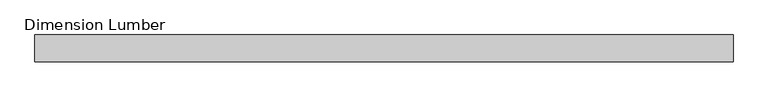
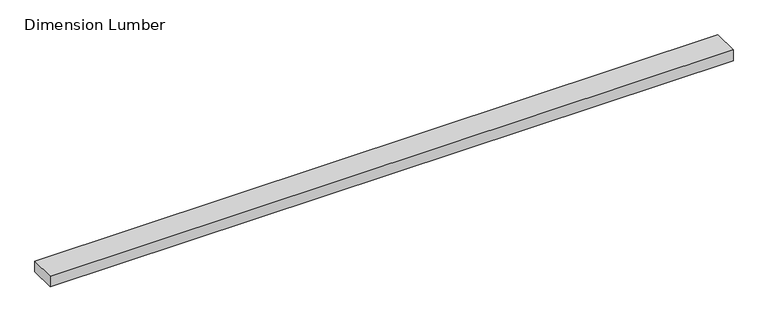
"""IFC4 building model written with IfcOpenShell, lengths in millimetres: beam geometry, Dimension Lumber : Top Supporting Lumbers."""

from ifc_helpers import new_model, si_unit, frame, origin, place, context, project, spatial, polyline, outline, extrude, source, transform, mapped, element, save


def dimension_lumber_7189ff9c(model_context):
    return source(origin(), model_context, "Body", "SweptSolid", [
        extrude(outline(polyline([(1146.96875, 44.45), (1146.96875, -44.45), (-1164.43125, -44.45), (-1164.43125, 44.45), (1146.96875, 44.45)])), frame((0.0, 0.0, -19.05), z_axis=(0.0, 0.0, 1.0), x_axis=(1.0, 0.0, 0.0)), (0.0, 0.0, 1.0), 38.1),
    ])


if __name__ == "__main__":
    model = new_model("IFC4")
    model_context = context("Model", 3, world=origin())
    ifc_project = project(units=[si_unit("LENGTHUNIT", "METRE", prefix="MILLI")], contexts=[model_context])
    site = spatial("IfcSite", under=ifc_project)
    building = spatial("IfcBuilding", under=site)
    placement = place(None, origin())
    dimension_lumber_shape = dimension_lumber_7189ff9c(model_context)
    element("IfcBeam", 1, ObjectType="Dimension Lumber : Top Supporting Lumbers", at=placement, inside=building, context=model_context, shape_type="MappedRepresentation", body=[
        mapped(dimension_lumber_shape, transform((0.0, 0.0, 0.0), x_axis=(1.0, 0.0, 0.0), y_axis=(0.0, 1.0, 0.0), z_axis=(0.0, 0.0, 1.0))),
    ])
    save(model, "model.ifc")

# Revit data of these elements
# Type "Dimension Lumber : Top Supporting Lumbers"
#   Assembly Code = "B10"
#   A = 0.0364583 SF
#   Length [instance default] = 5' - 0"
#   b = 0' - 3 1/2"
#   d = 0' - 1 1/2"
#   Structural Material [instance default] = Softwood, Lumber
# Element 1 (IfcBeam, "Dimension Lumber : Top Supporting Lumbers")
#   Structural Material = Douglas Fir #2
#   Materials on its faces: "Douglas Fir #2"
# Materials
#   "Softwood, Lumber": class "Wood", colour RGB 223 192 134, transparency 0, Description = "Pinus Echinata", Cost = 0
#   "Douglas Fir #2": class "Wood", colour RGB 223 192 134, transparency 0, Description = "Pinus Echinata", Cost = 0
